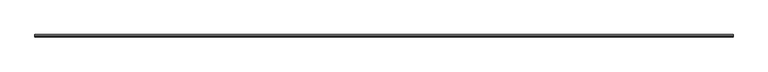
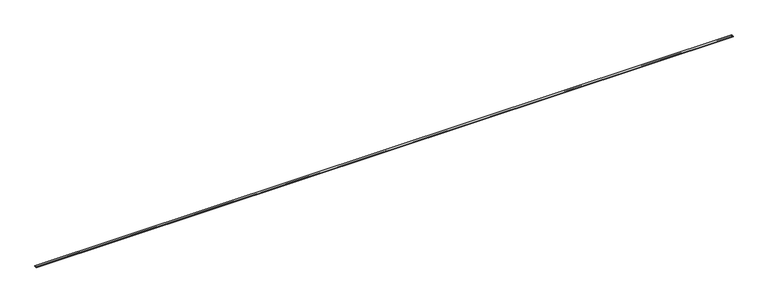
"""IFC4 building model written with IfcOpenShell, lengths in millimetres: proxy geometry, Generic Models 7:Generic Models 1:6:Generic Models 1:6 : Generic Models 7:Generic Models 1:337419:14 : Generic Models 7:Generic Models 1:6:Generic Models 1:6 : Generic Models 7:Generic Models 1:337419:312901."""

from ifc_helpers import new_model, si_unit, point, frame, frame_2d, origin, place, context, project, spatial, polyline, circle_curve, trimmed, segment, composite_curve, outline, extrude, source, transform, mapped, element, save


def generic_models_28b830fd(model_context):
    return source(origin(), model_context, "Body", "SweptSolid", [
        extrude(outline(polyline([(-578454.5913841, -63.5), (-578454.5913841, -165.1), (-578835.5913841, -165.1), (-578835.5913841, -63.5), (-578454.5913841, -63.5)]), holes=[composite_curve([segment(trimmed(circle_curve(frame_2d((-578733.9312882, -117.5511262)), 6.35), [point((-578727.5812882, -117.5511262))], [point((-578740.2812882, -117.5511262))], True, "CARTESIAN"), True, "CONTINUOUS"), segment(trimmed(circle_curve(frame_2d((-578733.9312882, -117.5511262)), 6.35), [point((-578740.2812882, -117.5511262))], [point((-578727.5812882, -117.5511262))], True, "CARTESIAN"), True, "CONTINUOUS")], self_intersect=False), composite_curve([segment(trimmed(circle_curve(frame_2d((-578632.3312882, -117.5511262)), 6.35), [point((-578625.9812882, -117.5511262))], [point((-578638.6812882, -117.5511262))], True, "CARTESIAN"), True, "CONTINUOUS"), segment(trimmed(circle_curve(frame_2d((-578632.3312882, -117.5511262)), 6.35), [point((-578638.6812882, -117.5511262))], [point((-578625.9812882, -117.5511262))], True, "CARTESIAN"), True, "CONTINUOUS")], self_intersect=False)]), frame((557771.6867239, 0.0, 0.0), z_axis=(1.0, 0.0, 0.0), x_axis=(0.0, 1.0, 0.0)), (0.0, 0.0, 1.0), 109559.725),
    ])


if __name__ == "__main__":
    model = new_model("IFC4")
    model_context = context("Model", 3, world=origin())
    ifc_project = project(units=[si_unit("LENGTHUNIT", "METRE", prefix="MILLI")], contexts=[model_context])
    site = spatial("IfcSite", under=ifc_project)
    building = spatial("IfcBuilding", under=site)
    placement = place(None, origin())
    generic_models_shape = generic_models_28b830fd(model_context)
    element("IfcBuildingElementProxy", 1, Name="Generic Models 7:Generic Models 1:6:Generic Models 1:6 : Generic Models 7:Generic Models 1:337419:14 : Generic Models 7:Generic Models 1:6:Generic Models 1:6 : Generic Models 7:Generic Models 1:337419:312901", ObjectType="Generic Models 7:Generic Models 1:6:Generic Models 1:6 : Generic Models 7:Generic Models 1:337419:14 : Generic Models 7:Generic Models 1:6:Generic Models 1:6 : Generic Models 7:Generic Models 1:337419:312901", at=placement, inside=building, context=model_context, shape_type="MappedRepresentation", body=[
        mapped(generic_models_shape, transform((0.0, 0.0, 0.0), x_axis=(1.0, 0.0, 0.0), y_axis=(0.0, 1.0, 0.0), z_axis=(0.0, 0.0, 1.0))),
    ])
    save(model, "model.ifc")

# Revit data of these elements
# Type "Generic Models 7:Generic Models 1:6:Generic Models 1:6 : Generic Models 7:Generic Models 1:337419:14 : Generic Models 7:Generic Models 1:6:Generic Models 1:6 : Generic Models 7:Generic Models 1:337419:312901"
#   NameOverride = "Generic Models 7:Generic Models 1:6:Generic Models 1:6 : Generic Models 7:Generic Models 1:337419:312901"
#   ObjectTypeOverride = "Generic Models 1:6 : Generic Models 7:Generic Models 1:337419"
#   Reference = "Generic Models 1"
#   Tag = "312901"
# Element 1 (IfcBuildingElementProxy, "Generic Models 7:Generic Models 1:6:Generic Models 1:6 : Generic Models 7:Generic Models 1:337419:14 : Generic Models 7:Generic Models 1:6:Generic Models 1:6 : Generic Models 7:Generic Models 1:337419:312901")
#   Materials on its faces: "CONCRETE SLAB - SEE STRUCT DWGS."
# Materials
#   "CONCRETE SLAB - SEE STRUCT DWGS.": class "Concrete", colour RGB 115 116 108, transparency 0, Description = "Lightweight concrete", Cost = 0
